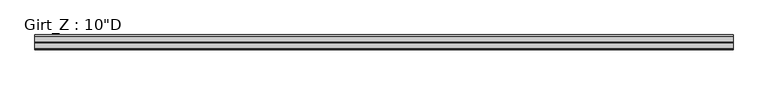
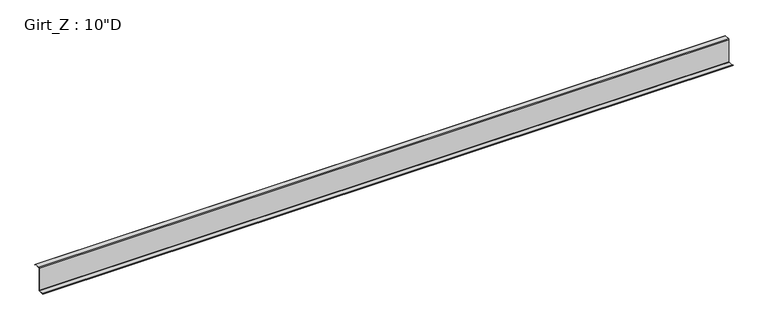
"""IFC4 building model written with IfcOpenShell, lengths in millimetres: beam geometry."""

from ifc_helpers import new_model, si_unit, point, frame, frame_2d, origin, place, context, project, spatial, polyline, circle_curve, trimmed, segment, composite_curve, outline, extrude, source, transform, mapped, element, save


def beam_dbcfb12a(model_context):
    return source(origin(), model_context, "Body", "SweptSolid", [
        extrude(outline(composite_curve([segment(polyline([(63.5, 127.0), (75.745104, 112.4068534), (73.6169367, 110.621109), (62.204539, 124.221875), (3.3005807, 124.221875)]), True, "CONTINUOUS"), segment(trimmed(circle_curve(frame_2d((3.3741066, 122.2381931)), 1.9850441), [point((3.3005807, 124.221875))], [point((1.3890625, 122.2381931))], True, "CARTESIAN"), True, "CONTINUOUS"), segment(polyline([(1.3890625, 122.2381931), (1.3890625, -122.2375)]), True, "CONTINUOUS"), segment(trimmed(circle_curve(frame_2d((-3.3734375, -122.2375)), 4.7625), [point((1.3890625, -122.2375))], [point((-3.3734375, -127.0))], False, "CARTESIAN"), True, "CONTINUOUS"), segment(polyline([(-3.3734375, -127.0), (-63.5, -127.0), (-75.745104, -112.4068534), (-73.6169367, -110.621109), (-62.204539, -124.221875), (-3.2694106, -124.221875)]), True, "CONTINUOUS"), segment(trimmed(circle_curve(frame_2d((-3.3748024, -122.2389339)), 1.9857399), [point((-3.2694106, -124.221875))], [point((-1.3890625, -122.2389339))], True, "CARTESIAN"), True, "CONTINUOUS"), segment(polyline([(-1.3890625, -122.2389339), (-1.3890625, 122.2375)]), True, "CONTINUOUS"), segment(trimmed(circle_curve(frame_2d((3.3734375, 122.2375)), 4.7625), [point((-1.3890625, 122.2375))], [point((3.3734375, 127.0))], False, "CARTESIAN"), True, "CONTINUOUS"), segment(polyline([(3.3734375, 127.0), (63.5, 127.0)]), True, "CONTINUOUS")], self_intersect=False)), frame((-3581.4, 0.0, 0.0), z_axis=(1.0, 0.0, 0.0), x_axis=(0.0, 1.0, 0.0)), (0.0, 0.0, 1.0), 7162.8),
    ])


if __name__ == "__main__":
    model = new_model("IFC4")
    model_context = context("Model", 3, world=origin())
    ifc_project = project(units=[si_unit("LENGTHUNIT", "METRE", prefix="MILLI")], contexts=[model_context])
    site = spatial("IfcSite", under=ifc_project)
    building = spatial("IfcBuilding", under=site)
    placement = place(None, origin())
    beam_shape = beam_dbcfb12a(model_context)
    element("IfcBeam", 1, ObjectType="Girt_Z : 10\"D", at=placement, inside=building, context=model_context, shape_type="MappedRepresentation", body=[
        mapped(beam_shape, transform((0.0, 0.0, 0.0), x_axis=(1.0, 0.0, 0.0), y_axis=(0.0, 1.0, 0.0), z_axis=(0.0, 0.0, 1.0))),
    ])
    save(model, "model.ifc")

# Revit data of these elements
# Type "Girt_Z : 10\"D"
#   Web_Thickness = 0' - 0 7/64"
#   Length [instance default] = 10' - 0"
#   Leg_1 = 0' - 2 1/2"
#   Height = 0' - 10"
#   Structural Material [instance default] = none
